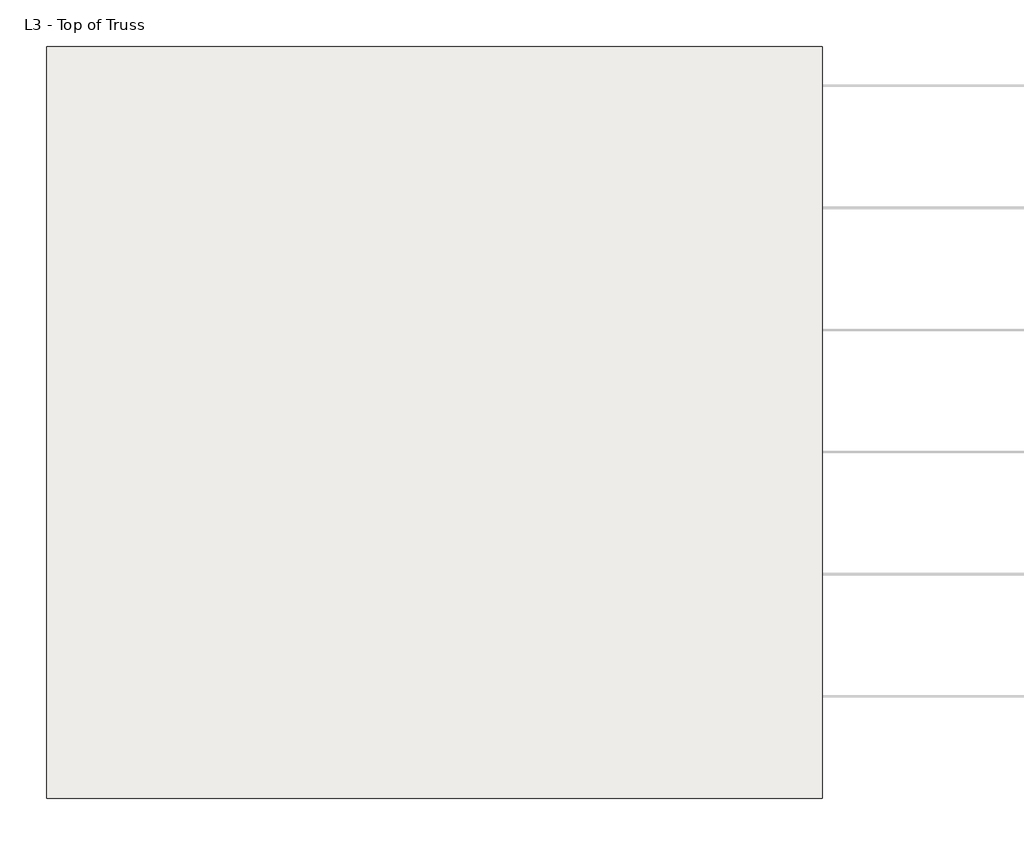
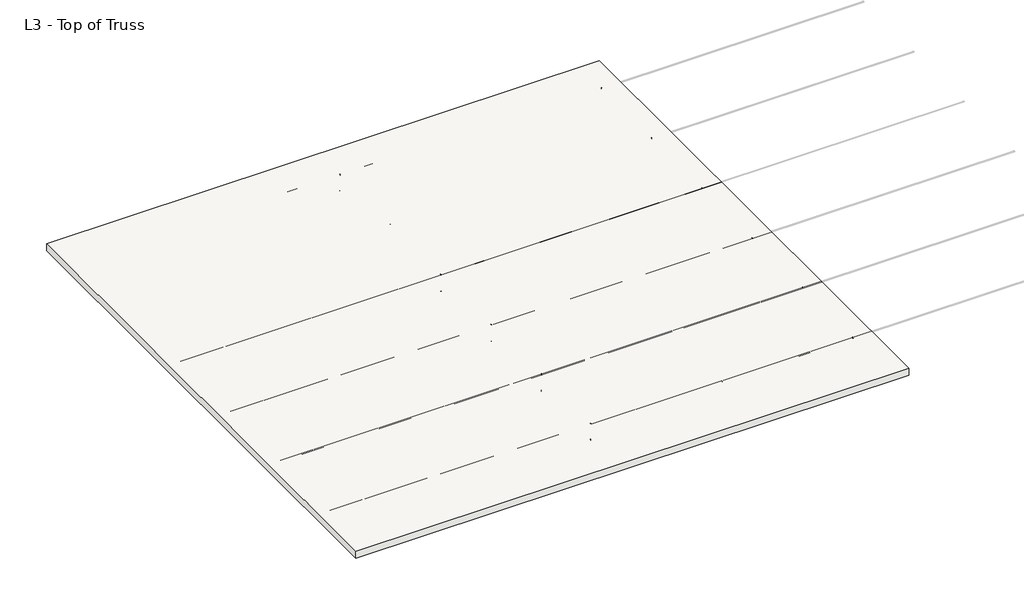
# One storey, part 1 of 2: 98 beams, 1 roof.
"""IFC4 building model written with IfcOpenShell, lengths in millimetres."""

import ifcopenshell
import ifcopenshell.guid

model = None  # the IFC model being written
_history = None  # IfcOwnerHistory: only IFC2X3 demands one
_inside = {}  # id of a spatial element -> (the spatial element, [elements in it])
_under = {}  # id of a project, library or spatial element -> (it, [spatial elements below it])
_declared = {}  # id of a project -> (the project, [libraries it declares])
_typed = {}  # id of a type object -> (the type object, [elements of that type])
_made_of = {}  # id of a material, layer set ... -> (it, [elements and type objects made of it])


def new_model(schema):
    """Start an empty IFC model of exactly this schema.

    Asked for "IFC4X3", IfcOpenShell would pick the latest addendum, in which some entities
    have other attributes; the version numbers below select the first issue.
    IFC2X3 requires an IfcOwnerHistory on every rooted entity: one is made here for all.
    """
    global model, _history
    if schema == "IFC4X3":
        model = ifcopenshell.file(schema_version=(4, 3, 0, 0))
    else:
        model = ifcopenshell.file(schema=schema)
    _inside.clear()
    _under.clear()
    _declared.clear()
    _typed.clear()
    _made_of.clear()
    _history = None
    if model.schema == "IFC2X3":
        org = make("IfcOrganization", Name="unknown")
        user = make(
            "IfcPersonAndOrganization",
            ThePerson=make("IfcPerson", FamilyName="unknown"),
            TheOrganization=org,
        )
        app = make(
            "IfcApplication",
            ApplicationDeveloper=org,
            Version="unknown",
            ApplicationFullName="unknown",
            ApplicationIdentifier="unknown",
        )
        _history = make(
            "IfcOwnerHistory",
            OwningUser=user,
            OwningApplication=app,
            ChangeAction="ADDED",
            CreationDate=0,
        )
    return model


def make(cls, **values):
    """One entity of the class cls with the attributes given. An attribute that is None is left unset."""
    return model.create_entity(
        cls, **{name: value for name, value in values.items() if value is not None}
    )


def rooted(cls, **values):
    """An entity with a GlobalId (a new one), such as an element, a storey or a relation."""
    return make(cls, GlobalId=ifcopenshell.guid.new(), OwnerHistory=_history, **values)


def si_unit(unit_type, name, prefix=None):
    """IfcSIUnit, for example si_unit("LENGTHUNIT", "METRE", prefix="MILLI")."""
    return make("IfcSIUnit", UnitType=unit_type, Prefix=prefix, Name=name)


def assignment(units):
    """IfcUnitAssignment: the units of a project."""
    return None if units is None else make("IfcUnitAssignment", Units=units)


def point(xyz):
    """IfcCartesianPoint."""
    return None if xyz is None else make("IfcCartesianPoint", Coordinates=xyz)


def direction(xyz):
    """IfcDirection."""
    return None if xyz is None else make("IfcDirection", DirectionRatios=xyz)


def frame(location, z_axis=None, x_axis=None):
    """IfcAxis2Placement3D, a coordinate frame: its origin and axes. An axis left out is left unset."""
    return make(
        "IfcAxis2Placement3D",
        Location=point(location),
        Axis=direction(z_axis),
        RefDirection=direction(x_axis),
    )


def frame_2d(location, x_axis=None):
    """IfcAxis2Placement2D, a coordinate frame in the plane: its origin and x axis."""
    return make(
        "IfcAxis2Placement2D", Location=point(location), RefDirection=direction(x_axis)
    )


def origin():
    """The frame at (0, 0, 0) with its axes left unset."""
    return frame((0.0, 0.0, 0.0))


def origin_2d():
    """The frame at (0, 0) in the plane with its x axis left unset."""
    return frame_2d((0.0, 0.0))


def place(relative_to, where):
    """IfcLocalPlacement: puts the frame where relative to a parent placement (None: the world)."""
    return make(
        "IfcLocalPlacement", PlacementRelTo=relative_to, RelativePlacement=where
    )


def context(
    kind, dimensions, precision=None, world=None, true_north=None, identifier=None
):
    """IfcGeometricRepresentationContext, for example the 3D "Model" context."""
    return make(
        "IfcGeometricRepresentationContext",
        ContextIdentifier=identifier,
        ContextType=kind,
        CoordinateSpaceDimension=dimensions,
        Precision=precision,
        WorldCoordinateSystem=world,
        TrueNorth=true_north,
    )


def project(units=None, contexts=None):
    """IfcProject with its units and contexts."""
    return rooted(
        "IfcProject",
        Name="project",
        RepresentationContexts=contexts,
        UnitsInContext=assignment(units),
    )


def spatial(cls, under=None, at=None, **own):
    """A site, building, storey or space (cls), placed at a placement, below another one or the project."""
    s = rooted(cls, ObjectPlacement=at, **own)
    if under is not None:
        _under.setdefault(under.id(), (under, []))[1].append(s)
    return s


def polyline(points):
    """IfcPolyline through the points."""
    return make("IfcPolyline", Points=[point(p) for p in points])


def circle_curve(where, radius):
    """IfcCircle in the frame where."""
    return make("IfcCircle", Position=where, Radius=radius)


def trimmed(basis, trim1, trim2, sense, master):
    """IfcTrimmedCurve: the piece of a basis curve between two trims."""
    return make(
        "IfcTrimmedCurve",
        BasisCurve=basis,
        Trim1=trim1,
        Trim2=trim2,
        SenseAgreement=sense,
        MasterRepresentation=master,
    )


def segment(curve, same_sense, transition):
    """IfcCompositeCurveSegment."""
    return make(
        "IfcCompositeCurveSegment",
        Transition=transition,
        SameSense=same_sense,
        ParentCurve=curve,
    )


def composite_curve(segments, self_intersect=None):
    """IfcCompositeCurve: segments joined end to end."""
    return make("IfcCompositeCurve", Segments=segments, SelfIntersect=self_intersect)


def outline(outer, holes=None, kind="AREA"):
    """IfcArbitraryClosedProfileDef: a profile drawn as a closed curve; with holes, ...WithVoids."""
    if holes is None:
        return make("IfcArbitraryClosedProfileDef", ProfileType=kind, OuterCurve=outer)
    return make(
        "IfcArbitraryProfileDefWithVoids",
        ProfileType=kind,
        OuterCurve=outer,
        InnerCurves=holes,
    )


def extrude(swept, where, along, depth):
    """IfcExtrudedAreaSolid: the profile swept, set in the frame where, extruded along a direction by depth."""
    return make(
        "IfcExtrudedAreaSolid",
        SweptArea=swept,
        Position=where,
        ExtrudedDirection=direction(along),
        Depth=depth,
    )


def shape(context_of_items, identifier, shape_type, items):
    """IfcShapeRepresentation: the items that make up one representation, for example the "Body"."""
    return make(
        "IfcShapeRepresentation",
        ContextOfItems=context_of_items,
        RepresentationIdentifier=identifier,
        RepresentationType=shape_type,
        Items=items,
    )


def source(mapping_origin, context_of_items, identifier, shape_type, items):
    """IfcRepresentationMap: a shape defined once, which mapped items show again and again."""
    return make(
        "IfcRepresentationMap",
        MappingOrigin=mapping_origin,
        MappedRepresentation=shape(context_of_items, identifier, shape_type, items),
    )


def transform(
    local_origin,
    x_axis=None,
    y_axis=None,
    z_axis=None,
    scale=None,
    scale2=None,
    scale3=None,
    uniform=True,
):
    """IfcCartesianTransformationOperator3D, or its non-uniform kind. x_axis, y_axis, z_axis: its Axis1, 2, 3."""
    if uniform:
        return make(
            "IfcCartesianTransformationOperator3D",
            Axis1=direction(x_axis),
            Axis2=direction(y_axis),
            LocalOrigin=point(local_origin),
            Scale=scale,
            Axis3=direction(z_axis),
        )
    return make(
        "IfcCartesianTransformationOperator3DnonUniform",
        Axis1=direction(x_axis),
        Axis2=direction(y_axis),
        LocalOrigin=point(local_origin),
        Scale=scale,
        Axis3=direction(z_axis),
        Scale2=scale2,
        Scale3=scale3,
    )


def mapped(mapping_source, mapping_target):
    """IfcMappedItem: shows the shape of a source again, moved by a transform."""
    return make(
        "IfcMappedItem", MappingSource=mapping_source, MappingTarget=mapping_target
    )


def made_of(thing, what):
    """Note that an element or type object is made of a material, layer set ...; save() writes the relation."""
    if what is not None:
        _made_of.setdefault(what.id(), (what, []))[1].append(thing)
    return thing


def element(
    cls,
    number,
    at=None,
    inside=None,
    cuts=None,
    type_object=None,
    material=None,
    context=None,
    identifier="Body",
    shape_type=None,
    held_by="IfcProductDefinitionShape",
    body=None,
    shapes=None,
    **own,
):
    """One element of the class cls, such as IfcWall. Its Tag is "e" and its number.

    at: its placement. inside: the storey or other place that contains it. cuts: it is an
    opening in that element (IfcRelVoidsElement). A single representation is given by context,
    identifier, shape_type and body (its items); several are given by shapes. held_by: the class
    of the entity that holds the representations. save() writes the other relations.
    """
    e = rooted(cls, Tag="e%d" % number, ObjectPlacement=at, **own)
    if body is not None:
        shapes = [shape(context, identifier, shape_type, body)]
    if shapes is not None:
        e.Representation = make(held_by, Representations=shapes)
    if inside is not None:
        _inside.setdefault(inside.id(), (inside, []))[1].append(e)
    if cuts is not None:
        rooted(
            "IfcRelVoidsElement", RelatingBuildingElement=cuts, RelatedOpeningElement=e
        )
    if type_object is not None:
        _typed.setdefault(type_object.id(), (type_object, []))[1].append(e)
    return made_of(e, material)


def aggregate(whole, parts):
    """IfcRelAggregates: a whole, such as a stair, and the parts it consists of."""
    return rooted("IfcRelAggregates", RelatingObject=whole, RelatedObjects=parts)


def save(model, path):
    """Write the relations noted so far, then the file.

    IfcRelAggregates (storeys below a building ...), IfcRelContainedInSpatialStructure (elements
    in a storey), IfcRelDefinesByType, IfcRelAssociatesMaterial and IfcRelDeclares: one each for
    every whole, place, type object, material and project.
    """
    for whole, parts in _under.values():
        aggregate(whole, parts)
    for where, things in _inside.values():
        rooted(
            "IfcRelContainedInSpatialStructure",
            RelatedElements=things,
            RelatingStructure=where,
        )
    for kind, things in _typed.values():
        rooted("IfcRelDefinesByType", RelatedObjects=things, RelatingType=kind)
    for what, things in _made_of.values():
        rooted("IfcRelAssociatesMaterial", RelatedObjects=things, RelatingMaterial=what)
    for by, libraries in _declared.values():
        rooted("IfcRelDeclares", RelatingContext=by, RelatedDefinitions=libraries)
    model.write(path)


def circular_hollow_sections_chs60_3x5_c94bd862(model_context):
    return source(origin(), model_context, "Body", "SweptSolid", [
        extrude(outline(composite_curve([segment(trimmed(circle_curve(origin_2d(), 30.15), [point((-30.15, 0.0))], [point((30.15, 0.0))], False, "CARTESIAN"), True, "CONTINUOUS"), segment(trimmed(circle_curve(origin_2d(), 30.15), [point((30.15, 0.0))], [point((-30.15, 0.0))], False, "CARTESIAN"), True, "CONTINUOUS")], self_intersect=False), holes=[composite_curve([segment(trimmed(circle_curve(origin_2d(), 25.15), [point((25.15, 0.0))], [point((-25.15, 0.0))], True, "CARTESIAN"), True, "CONTINUOUS"), segment(trimmed(circle_curve(origin_2d(), 25.15), [point((-25.15, 0.0))], [point((25.15, 0.0))], True, "CARTESIAN"), True, "CONTINUOUS")], self_intersect=False)]), frame((-557.0, 0.0, 0.0), z_axis=(1.0, 0.0, 0.0), x_axis=(0.0, 1.0, 0.0)), (0.0, 0.0, 1.0), 1114.0),
    ])


def circular_hollow_sections_chs60_3x5_b8a643cb(model_context):
    return source(origin(), model_context, "Body", "SweptSolid", [
        extrude(outline(composite_curve([segment(trimmed(circle_curve(origin_2d(), 30.15), [point((-30.15, 0.0))], [point((30.15, 0.0))], False, "CARTESIAN"), True, "CONTINUOUS"), segment(trimmed(circle_curve(origin_2d(), 30.15), [point((30.15, 0.0))], [point((-30.15, 0.0))], False, "CARTESIAN"), True, "CONTINUOUS")], self_intersect=False), holes=[composite_curve([segment(trimmed(circle_curve(origin_2d(), 25.15), [point((25.15, 0.0))], [point((-25.15, 0.0))], True, "CARTESIAN"), True, "CONTINUOUS"), segment(trimmed(circle_curve(origin_2d(), 25.15), [point((-25.15, 0.0))], [point((25.15, 0.0))], True, "CARTESIAN"), True, "CONTINUOUS")], self_intersect=False)]), frame((-790.0, 0.0, 0.0), z_axis=(1.0, 0.0, 0.0), x_axis=(0.0, 1.0, 0.0)), (0.0, 0.0, 1.0), 1580.0),
    ])


def circular_hollow_sections_chs60_3x5_ee2473de(model_context):
    return source(origin(), model_context, "Body", "SweptSolid", [
        extrude(outline(composite_curve([segment(trimmed(circle_curve(origin_2d(), 30.15), [point((-30.15, 0.0))], [point((30.15, 0.0))], False, "CARTESIAN"), True, "CONTINUOUS"), segment(trimmed(circle_curve(origin_2d(), 30.15), [point((30.15, 0.0))], [point((-30.15, 0.0))], False, "CARTESIAN"), True, "CONTINUOUS")], self_intersect=False), holes=[composite_curve([segment(trimmed(circle_curve(origin_2d(), 25.15), [point((25.15, 0.0))], [point((-25.15, 0.0))], True, "CARTESIAN"), True, "CONTINUOUS"), segment(trimmed(circle_curve(origin_2d(), 25.15), [point((-25.15, 0.0))], [point((25.15, 0.0))], True, "CARTESIAN"), True, "CONTINUOUS")], self_intersect=False)]), frame((-9000.0, 0.0, 0.0), z_axis=(1.0, 0.0, 0.0), x_axis=(0.0, 1.0, 0.0)), (0.0, 0.0, 1.0), 18000.0),
    ])


def circular_hollow_sections_chs60_3x5_7809bf4e(model_context):
    return source(origin(), model_context, "Body", "SweptSolid", [
        extrude(outline(composite_curve([segment(trimmed(circle_curve(origin_2d(), 30.15), [point((-30.15, 0.0))], [point((30.15, 0.0))], False, "CARTESIAN"), True, "CONTINUOUS"), segment(trimmed(circle_curve(origin_2d(), 30.15), [point((30.15, 0.0))], [point((-30.15, 0.0))], False, "CARTESIAN"), True, "CONTINUOUS")], self_intersect=False), holes=[composite_curve([segment(trimmed(circle_curve(origin_2d(), 25.15), [point((25.15, 0.0))], [point((-25.15, 0.0))], True, "CARTESIAN"), True, "CONTINUOUS"), segment(trimmed(circle_curve(origin_2d(), 25.15), [point((-25.15, 0.0))], [point((25.15, 0.0))], True, "CARTESIAN"), True, "CONTINUOUS")], self_intersect=False)]), frame((-600.0, 0.0, 0.0), z_axis=(1.0, 0.0, 0.0), x_axis=(0.0, 1.0, 0.0)), (0.0, 0.0, 1.0), 1157.0),
    ])


model = new_model("IFC4")

# Units and contexts
model_context = context("Model", 3, world=origin())
ifc_project = project(units=[si_unit("LENGTHUNIT", "METRE", prefix="MILLI")], contexts=[model_context])

# Site, building, storey
site = spatial("IfcSite", under=ifc_project)
building = spatial("IfcBuilding", under=site)
storey = spatial("IfcBuildingStorey", under=building, Name="L3 - Top of Truss", Elevation=7800.0)

# Beams
placement = place(None, origin())
circular_hollow_sections_chs60_3x5_shape = circular_hollow_sections_chs60_3x5_c94bd862(model_context)
element("IfcBeam", 1, ObjectType="Circular Hollow Sections : CHS60.3x5", at=placement, inside=storey, context=model_context, shape_type="MappedRepresentation", body=[
    mapped(circular_hollow_sections_chs60_3x5_shape, transform((-5853.84106, -5058.7619082, 7200.0), x_axis=(0.0, 0.0, 1.0), y_axis=(0.0, -1.0, 0.0), z_axis=(1.0, 0.0, 0.0))),
])
element("IfcBeam", 2, ObjectType="Circular Hollow Sections : CHS60.3x5", at=placement, inside=storey, context=model_context, shape_type="MappedRepresentation", body=[
    mapped(circular_hollow_sections_chs60_3x5_shape, transform((-4568.1267743, -5058.7619082, 7200.0), x_axis=(0.0, 0.0, 1.0), y_axis=(0.0, -1.0, 0.0), z_axis=(1.0, 0.0, 0.0))),
])
element("IfcBeam", 3, ObjectType="Circular Hollow Sections : CHS60.3x5", at=placement, inside=storey, context=model_context, shape_type="MappedRepresentation", body=[
    mapped(circular_hollow_sections_chs60_3x5_shape, transform((-3282.4124885, -5058.7619082, 7200.0), x_axis=(0.0, 0.0, 1.0), y_axis=(0.0, -1.0, 0.0), z_axis=(1.0, 0.0, 0.0))),
])
element("IfcBeam", 4, ObjectType="Circular Hollow Sections : CHS60.3x5", at=placement, inside=storey, context=model_context, shape_type="MappedRepresentation", body=[
    mapped(circular_hollow_sections_chs60_3x5_shape, transform((-1996.6982028, -5058.7619082, 7200.0), x_axis=(0.0, 0.0, 1.0), y_axis=(0.0, -1.0, 0.0), z_axis=(1.0, 0.0, 0.0))),
])
element("IfcBeam", 5, ObjectType="Circular Hollow Sections : CHS60.3x5", at=placement, inside=storey, context=model_context, shape_type="MappedRepresentation", body=[
    mapped(circular_hollow_sections_chs60_3x5_shape, transform((-710.9839171, -5058.7619082, 7200.0), x_axis=(0.0, 0.0, 1.0), y_axis=(0.0, -1.0, 0.0), z_axis=(1.0, 0.0, 0.0))),
])
element("IfcBeam", 6, ObjectType="Circular Hollow Sections : CHS60.3x5", at=placement, inside=storey, context=model_context, shape_type="MappedRepresentation", body=[
    mapped(circular_hollow_sections_chs60_3x5_shape, transform((-5853.84106, -11058.7619082, 7200.0), x_axis=(0.0, 0.0, 1.0), y_axis=(0.0, -1.0, 0.0), z_axis=(1.0, 0.0, 0.0))),
])
element("IfcBeam", 7, ObjectType="Circular Hollow Sections : CHS60.3x5", at=placement, inside=storey, context=model_context, shape_type="MappedRepresentation", body=[
    mapped(circular_hollow_sections_chs60_3x5_shape, transform((-4568.1267743, -11058.7619082, 7200.0), x_axis=(0.0, 0.0, 1.0), y_axis=(0.0, -1.0, 0.0), z_axis=(1.0, 0.0, 0.0))),
])
element("IfcBeam", 8, ObjectType="Circular Hollow Sections : CHS60.3x5", at=placement, inside=storey, context=model_context, shape_type="MappedRepresentation", body=[
    mapped(circular_hollow_sections_chs60_3x5_shape, transform((-3282.4124885, -11058.7619082, 7200.0), x_axis=(0.0, 0.0, 1.0), y_axis=(0.0, -1.0, 0.0), z_axis=(1.0, 0.0, 0.0))),
])
element("IfcBeam", 9, ObjectType="Circular Hollow Sections : CHS60.3x5", at=placement, inside=storey, context=model_context, shape_type="MappedRepresentation", body=[
    mapped(circular_hollow_sections_chs60_3x5_shape, transform((5717.5875115, -11058.7619082, 7200.0), x_axis=(0.0, 0.0, 1.0), y_axis=(0.0, -1.0, 0.0), z_axis=(1.0, 0.0, 0.0))),
])
element("IfcBeam", 10, ObjectType="Circular Hollow Sections : CHS60.3x5", at=placement, inside=storey, context=model_context, shape_type="MappedRepresentation", body=[
    mapped(circular_hollow_sections_chs60_3x5_shape, transform((4431.8732257, -11058.7619082, 7200.0), x_axis=(0.0, 0.0, 1.0), y_axis=(0.0, -1.0, 0.0), z_axis=(1.0, 0.0, 0.0))),
])
element("IfcBeam", 11, ObjectType="Circular Hollow Sections : CHS60.3x5", at=placement, inside=storey, context=model_context, shape_type="MappedRepresentation", body=[
    mapped(circular_hollow_sections_chs60_3x5_shape, transform((3146.15894, -11058.7619082, 7200.0), x_axis=(0.0, 0.0, 1.0), y_axis=(0.0, -1.0, 0.0), z_axis=(1.0, 0.0, 0.0))),
])
element("IfcBeam", 12, ObjectType="Circular Hollow Sections : CHS60.3x5", at=placement, inside=storey, context=model_context, shape_type="MappedRepresentation", body=[
    mapped(circular_hollow_sections_chs60_3x5_shape, transform((-1996.6982028, -11058.7619082, 7200.0), x_axis=(0.0, 0.0, 1.0), y_axis=(0.0, -1.0, 0.0), z_axis=(1.0, 0.0, 0.0))),
])
element("IfcBeam", 13, ObjectType="Circular Hollow Sections : CHS60.3x5", at=placement, inside=storey, context=model_context, shape_type="MappedRepresentation", body=[
    mapped(circular_hollow_sections_chs60_3x5_shape, transform((-710.9839171, -11058.7619082, 7200.0), x_axis=(0.0, 0.0, 1.0), y_axis=(0.0, -1.0, 0.0), z_axis=(1.0, 0.0, 0.0))),
])
element("IfcBeam", 14, ObjectType="Circular Hollow Sections : CHS60.3x5", at=placement, inside=storey, context=model_context, shape_type="MappedRepresentation", body=[
    mapped(circular_hollow_sections_chs60_3x5_shape, transform((574.7303686, -11058.7619082, 7200.0), x_axis=(0.0, 0.0, 1.0), y_axis=(0.0, -1.0, 0.0), z_axis=(1.0, 0.0, 0.0))),
])
element("IfcBeam", 15, ObjectType="Circular Hollow Sections : CHS60.3x5", at=placement, inside=storey, context=model_context, shape_type="MappedRepresentation", body=[
    mapped(circular_hollow_sections_chs60_3x5_shape, transform((1860.4446543, -11058.7619082, 7200.0), x_axis=(0.0, 0.0, 1.0), y_axis=(0.0, -1.0, 0.0), z_axis=(1.0, 0.0, 0.0))),
])
element("IfcBeam", 16, ObjectType="Circular Hollow Sections : CHS60.3x5", at=placement, inside=storey, context=model_context, shape_type="MappedRepresentation", body=[
    mapped(circular_hollow_sections_chs60_3x5_shape, transform((9574.7303686, -17058.7619082, 7200.0), x_axis=(0.0, 0.0, 1.0), y_axis=(0.0, -1.0, 0.0), z_axis=(1.0, 0.0, 0.0))),
])
element("IfcBeam", 17, ObjectType="Circular Hollow Sections : CHS60.3x5", at=placement, inside=storey, context=model_context, shape_type="MappedRepresentation", body=[
    mapped(circular_hollow_sections_chs60_3x5_shape, transform((-5853.84106, -17058.7619082, 7200.0), x_axis=(0.0, 0.0, 1.0), y_axis=(0.0, -1.0, 0.0), z_axis=(1.0, 0.0, 0.0))),
])
element("IfcBeam", 18, ObjectType="Circular Hollow Sections : CHS60.3x5", at=placement, inside=storey, context=model_context, shape_type="MappedRepresentation", body=[
    mapped(circular_hollow_sections_chs60_3x5_shape, transform((8289.0160829, -17058.7619082, 7200.0), x_axis=(0.0, 0.0, 1.0), y_axis=(0.0, -1.0, 0.0), z_axis=(1.0, 0.0, 0.0))),
])
element("IfcBeam", 19, ObjectType="Circular Hollow Sections : CHS60.3x5", at=placement, inside=storey, context=model_context, shape_type="MappedRepresentation", body=[
    mapped(circular_hollow_sections_chs60_3x5_shape, transform((-4568.1267743, -17058.7619082, 7200.0), x_axis=(0.0, 0.0, 1.0), y_axis=(0.0, -1.0, 0.0), z_axis=(1.0, 0.0, 0.0))),
])
element("IfcBeam", 20, ObjectType="Circular Hollow Sections : CHS60.3x5", at=placement, inside=storey, context=model_context, shape_type="MappedRepresentation", body=[
    mapped(circular_hollow_sections_chs60_3x5_shape, transform((7003.3017972, -17058.7619082, 7200.0), x_axis=(0.0, 0.0, 1.0), y_axis=(0.0, -1.0, 0.0), z_axis=(1.0, 0.0, 0.0))),
])
element("IfcBeam", 21, ObjectType="Circular Hollow Sections : CHS60.3x5", at=placement, inside=storey, context=model_context, shape_type="MappedRepresentation", body=[
    mapped(circular_hollow_sections_chs60_3x5_shape, transform((-3282.4124885, -17058.7619082, 7200.0), x_axis=(0.0, 0.0, 1.0), y_axis=(0.0, -1.0, 0.0), z_axis=(1.0, 0.0, 0.0))),
])
element("IfcBeam", 22, ObjectType="Circular Hollow Sections : CHS60.3x5", at=placement, inside=storey, context=model_context, shape_type="MappedRepresentation", body=[
    mapped(circular_hollow_sections_chs60_3x5_shape, transform((5717.5875115, -17058.7619082, 7200.0), x_axis=(0.0, 0.0, 1.0), y_axis=(0.0, -1.0, 0.0), z_axis=(1.0, 0.0, 0.0))),
])
element("IfcBeam", 23, ObjectType="Circular Hollow Sections : CHS60.3x5", at=placement, inside=storey, context=model_context, shape_type="MappedRepresentation", body=[
    mapped(circular_hollow_sections_chs60_3x5_shape, transform((4431.8732257, -17058.7619082, 7200.0), x_axis=(0.0, 0.0, 1.0), y_axis=(0.0, -1.0, 0.0), z_axis=(1.0, 0.0, 0.0))),
])
element("IfcBeam", 24, ObjectType="Circular Hollow Sections : CHS60.3x5", at=placement, inside=storey, context=model_context, shape_type="MappedRepresentation", body=[
    mapped(circular_hollow_sections_chs60_3x5_shape, transform((3146.15894, -17058.7619082, 7200.0), x_axis=(0.0, 0.0, 1.0), y_axis=(0.0, -1.0, 0.0), z_axis=(1.0, 0.0, 0.0))),
])
element("IfcBeam", 25, ObjectType="Circular Hollow Sections : CHS60.3x5", at=placement, inside=storey, context=model_context, shape_type="MappedRepresentation", body=[
    mapped(circular_hollow_sections_chs60_3x5_shape, transform((-1996.6982028, -17058.7619082, 7200.0), x_axis=(0.0, 0.0, 1.0), y_axis=(0.0, -1.0, 0.0), z_axis=(1.0, 0.0, 0.0))),
])
element("IfcBeam", 26, ObjectType="Circular Hollow Sections : CHS60.3x5", at=placement, inside=storey, context=model_context, shape_type="MappedRepresentation", body=[
    mapped(circular_hollow_sections_chs60_3x5_shape, transform((-710.9839171, -17058.7619082, 7200.0), x_axis=(0.0, 0.0, 1.0), y_axis=(0.0, -1.0, 0.0), z_axis=(1.0, 0.0, 0.0))),
])
element("IfcBeam", 27, ObjectType="Circular Hollow Sections : CHS60.3x5", at=placement, inside=storey, context=model_context, shape_type="MappedRepresentation", body=[
    mapped(circular_hollow_sections_chs60_3x5_shape, transform((574.7303686, -17058.7619082, 7200.0), x_axis=(0.0, 0.0, 1.0), y_axis=(0.0, -1.0, 0.0), z_axis=(1.0, 0.0, 0.0))),
])
element("IfcBeam", 28, ObjectType="Circular Hollow Sections : CHS60.3x5", at=placement, inside=storey, context=model_context, shape_type="MappedRepresentation", body=[
    mapped(circular_hollow_sections_chs60_3x5_shape, transform((1860.4446543, -17058.7619082, 7200.0), x_axis=(0.0, 0.0, 1.0), y_axis=(0.0, -1.0, 0.0), z_axis=(1.0, 0.0, 0.0))),
])
element("IfcBeam", 29, ObjectType="Circular Hollow Sections : CHS60.3x5", at=placement, inside=storey, context=model_context, shape_type="MappedRepresentation", body=[
    mapped(circular_hollow_sections_chs60_3x5_shape, transform((9574.7303686, -22948.7619082, 7200.0), x_axis=(0.0, 0.0, 1.0), y_axis=(0.0, -1.0, 0.0), z_axis=(1.0, 0.0, 0.0))),
])
element("IfcBeam", 30, ObjectType="Circular Hollow Sections : CHS60.3x5", at=placement, inside=storey, context=model_context, shape_type="MappedRepresentation", body=[
    mapped(circular_hollow_sections_chs60_3x5_shape, transform((-5853.84106, -22948.7619082, 7200.0), x_axis=(0.0, 0.0, 1.0), y_axis=(0.0, -1.0, 0.0), z_axis=(1.0, 0.0, 0.0))),
])
element("IfcBeam", 31, ObjectType="Circular Hollow Sections : CHS60.3x5", at=placement, inside=storey, context=model_context, shape_type="MappedRepresentation", body=[
    mapped(circular_hollow_sections_chs60_3x5_shape, transform((8289.0160829, -22948.7619082, 7200.0), x_axis=(0.0, 0.0, 1.0), y_axis=(0.0, -1.0, 0.0), z_axis=(1.0, 0.0, 0.0))),
])
element("IfcBeam", 32, ObjectType="Circular Hollow Sections : CHS60.3x5", at=placement, inside=storey, context=model_context, shape_type="MappedRepresentation", body=[
    mapped(circular_hollow_sections_chs60_3x5_shape, transform((-4568.1267743, -22948.7619082, 7200.0), x_axis=(0.0, 0.0, 1.0), y_axis=(0.0, -1.0, 0.0), z_axis=(1.0, 0.0, 0.0))),
])
element("IfcBeam", 33, ObjectType="Circular Hollow Sections : CHS60.3x5", at=placement, inside=storey, context=model_context, shape_type="MappedRepresentation", body=[
    mapped(circular_hollow_sections_chs60_3x5_shape, transform((7003.3017972, -22948.7619082, 7200.0), x_axis=(0.0, 0.0, 1.0), y_axis=(0.0, -1.0, 0.0), z_axis=(1.0, 0.0, 0.0))),
])
element("IfcBeam", 34, ObjectType="Circular Hollow Sections : CHS60.3x5", at=placement, inside=storey, context=model_context, shape_type="MappedRepresentation", body=[
    mapped(circular_hollow_sections_chs60_3x5_shape, transform((-3282.4124885, -22948.7619082, 7200.0), x_axis=(0.0, 0.0, 1.0), y_axis=(0.0, -1.0, 0.0), z_axis=(1.0, 0.0, 0.0))),
])
element("IfcBeam", 35, ObjectType="Circular Hollow Sections : CHS60.3x5", at=placement, inside=storey, context=model_context, shape_type="MappedRepresentation", body=[
    mapped(circular_hollow_sections_chs60_3x5_shape, transform((5717.5875115, -22948.7619082, 7200.0), x_axis=(0.0, 0.0, 1.0), y_axis=(0.0, -1.0, 0.0), z_axis=(1.0, 0.0, 0.0))),
])
element("IfcBeam", 36, ObjectType="Circular Hollow Sections : CHS60.3x5", at=placement, inside=storey, context=model_context, shape_type="MappedRepresentation", body=[
    mapped(circular_hollow_sections_chs60_3x5_shape, transform((4431.8732257, -22948.7619082, 7200.0), x_axis=(0.0, 0.0, 1.0), y_axis=(0.0, -1.0, 0.0), z_axis=(1.0, 0.0, 0.0))),
])
element("IfcBeam", 37, ObjectType="Circular Hollow Sections : CHS60.3x5", at=placement, inside=storey, context=model_context, shape_type="MappedRepresentation", body=[
    mapped(circular_hollow_sections_chs60_3x5_shape, transform((10860.4446543, -22948.7619082, 7200.0), x_axis=(0.0, 0.0, 1.0), y_axis=(0.0, -1.0, 0.0), z_axis=(1.0, 0.0, 0.0))),
])
element("IfcBeam", 38, ObjectType="Circular Hollow Sections : CHS60.3x5", at=placement, inside=storey, context=model_context, shape_type="MappedRepresentation", body=[
    mapped(circular_hollow_sections_chs60_3x5_shape, transform((3146.15894, -22948.7619082, 7200.0), x_axis=(0.0, 0.0, 1.0), y_axis=(0.0, -1.0, 0.0), z_axis=(1.0, 0.0, 0.0))),
])
element("IfcBeam", 39, ObjectType="Circular Hollow Sections : CHS60.3x5", at=placement, inside=storey, context=model_context, shape_type="MappedRepresentation", body=[
    mapped(circular_hollow_sections_chs60_3x5_shape, transform((-1996.6982028, -22948.7619082, 7200.0), x_axis=(0.0, 0.0, 1.0), y_axis=(0.0, -1.0, 0.0), z_axis=(1.0, 0.0, 0.0))),
])
element("IfcBeam", 40, ObjectType="Circular Hollow Sections : CHS60.3x5", at=placement, inside=storey, context=model_context, shape_type="MappedRepresentation", body=[
    mapped(circular_hollow_sections_chs60_3x5_shape, transform((-710.9839171, -22948.7619082, 7200.0), x_axis=(0.0, 0.0, 1.0), y_axis=(0.0, -1.0, 0.0), z_axis=(1.0, 0.0, 0.0))),
])
element("IfcBeam", 41, ObjectType="Circular Hollow Sections : CHS60.3x5", at=placement, inside=storey, context=model_context, shape_type="MappedRepresentation", body=[
    mapped(circular_hollow_sections_chs60_3x5_shape, transform((-7139.5553457, -22948.7619082, 7200.0), x_axis=(0.0, 0.0, 1.0), y_axis=(0.0, -1.0, 0.0), z_axis=(1.0, 0.0, 0.0))),
])
element("IfcBeam", 42, ObjectType="Circular Hollow Sections : CHS60.3x5", at=placement, inside=storey, context=model_context, shape_type="MappedRepresentation", body=[
    mapped(circular_hollow_sections_chs60_3x5_shape, transform((574.7303686, -22948.7619082, 7200.0), x_axis=(0.0, 0.0, 1.0), y_axis=(0.0, -1.0, 0.0), z_axis=(1.0, 0.0, 0.0))),
])
element("IfcBeam", 43, ObjectType="Circular Hollow Sections : CHS60.3x5", at=placement, inside=storey, context=model_context, shape_type="MappedRepresentation", body=[
    mapped(circular_hollow_sections_chs60_3x5_shape, transform((1860.4446543, -22948.7619082, 7200.0), x_axis=(0.0, 0.0, 1.0), y_axis=(0.0, -1.0, 0.0), z_axis=(1.0, 0.0, 0.0))),
])
circular_hollow_sections_chs60_3x5_2_shape = circular_hollow_sections_chs60_3x5_b8a643cb(model_context)
element("IfcBeam", 44, ObjectType="Circular Hollow Sections : CHS60.3x5", at=placement, inside=storey, context=model_context, shape_type="MappedRepresentation", body=[
    mapped(circular_hollow_sections_chs60_3x5_2_shape, transform((-5210.9839171, -5058.7619082, 7200.0), x_axis=(0.7310552682428689, 0.0, -0.6823182503600113), y_axis=(0.0, -1.0, 0.0), z_axis=(-0.6823182503600113, 0.0, -0.7310552682428689))),
])
element("IfcBeam", 45, ObjectType="Circular Hollow Sections : CHS60.3x5", at=placement, inside=storey, context=model_context, shape_type="MappedRepresentation", body=[
    mapped(circular_hollow_sections_chs60_3x5_2_shape, transform((-3925.2696314, -5058.7619082, 7200.0), x_axis=(0.7310552682428689, 0.0, -0.6823182503600113), y_axis=(0.0, -1.0, 0.0), z_axis=(-0.6823182503600113, 0.0, -0.7310552682428689))),
])
element("IfcBeam", 46, ObjectType="Circular Hollow Sections : CHS60.3x5", at=placement, inside=storey, context=model_context, shape_type="MappedRepresentation", body=[
    mapped(circular_hollow_sections_chs60_3x5_2_shape, transform((-2639.5553457, -5058.7619082, 7200.0), x_axis=(0.7310552682428689, 0.0, -0.6823182503600113), y_axis=(0.0, -1.0, 0.0), z_axis=(-0.6823182503600113, 0.0, -0.7310552682428689))),
])
element("IfcBeam", 47, ObjectType="Circular Hollow Sections : CHS60.3x5", at=placement, inside=storey, context=model_context, shape_type="MappedRepresentation", body=[
    mapped(circular_hollow_sections_chs60_3x5_2_shape, transform((-1353.84106, -5058.7619082, 7200.0), x_axis=(0.7310552682428689, 0.0, -0.6823182503600113), y_axis=(0.0, -1.0, 0.0), z_axis=(-0.6823182503600113, 0.0, -0.7310552682428689))),
])
element("IfcBeam", 48, ObjectType="Circular Hollow Sections : CHS60.3x5", at=placement, inside=storey, context=model_context, shape_type="MappedRepresentation", body=[
    mapped(circular_hollow_sections_chs60_3x5_2_shape, transform((-68.1267743, -5058.7619082, 7200.0), x_axis=(0.7310552682428689, 0.0, -0.6823182503600113), y_axis=(0.0, -1.0, 0.0), z_axis=(-0.6823182503600113, 0.0, -0.7310552682428689))),
])
element("IfcBeam", 49, ObjectType="Circular Hollow Sections : CHS60.3x5", at=placement, inside=storey, context=model_context, shape_type="MappedRepresentation", body=[
    mapped(circular_hollow_sections_chs60_3x5_2_shape, transform((-6496.6982028, -5058.7619082, 7200.0), x_axis=(0.7310552682428691, 0.0, -0.6823182503600111), y_axis=(0.0, -1.0, 0.0), z_axis=(-0.6823182503600111, 0.0, -0.7310552682428691))),
])
element("IfcBeam", 50, ObjectType="Circular Hollow Sections : CHS60.3x5", at=placement, inside=storey, context=model_context, shape_type="MappedRepresentation", body=[
    mapped(circular_hollow_sections_chs60_3x5_2_shape, transform((-5210.9839171, -11058.7619082, 7200.0), x_axis=(0.7310552682428689, 0.0, -0.6823182503600113), y_axis=(0.0, -1.0, 0.0), z_axis=(-0.6823182503600113, 0.0, -0.7310552682428689))),
])
element("IfcBeam", 51, ObjectType="Circular Hollow Sections : CHS60.3x5", at=placement, inside=storey, context=model_context, shape_type="MappedRepresentation", body=[
    mapped(circular_hollow_sections_chs60_3x5_2_shape, transform((-3925.2696314, -11058.7619082, 7200.0), x_axis=(0.7310552682428689, 0.0, -0.6823182503600113), y_axis=(0.0, -1.0, 0.0), z_axis=(-0.6823182503600113, 0.0, -0.7310552682428689))),
])
element("IfcBeam", 52, ObjectType="Circular Hollow Sections : CHS60.3x5", at=placement, inside=storey, context=model_context, shape_type="MappedRepresentation", body=[
    mapped(circular_hollow_sections_chs60_3x5_2_shape, transform((-2639.5553457, -11058.7619082, 7200.0), x_axis=(0.7310552682428689, 0.0, -0.6823182503600113), y_axis=(0.0, -1.0, 0.0), z_axis=(-0.6823182503600113, 0.0, -0.7310552682428689))),
])
element("IfcBeam", 53, ObjectType="Circular Hollow Sections : CHS60.3x5", at=placement, inside=storey, context=model_context, shape_type="MappedRepresentation", body=[
    mapped(circular_hollow_sections_chs60_3x5_2_shape, transform((3789.0160829, -11058.7619082, 7200.0), x_axis=(0.7310552682428691, 0.0, 0.6823182503600111), y_axis=(0.0, -1.0, 0.0), z_axis=(0.6823182503600111, 0.0, -0.7310552682428691))),
])
element("IfcBeam", 54, ObjectType="Circular Hollow Sections : CHS60.3x5", at=placement, inside=storey, context=model_context, shape_type="MappedRepresentation", body=[
    mapped(circular_hollow_sections_chs60_3x5_2_shape, transform((2503.3017972, -11058.7619082, 7200.0), x_axis=(0.7310552682428691, 0.0, 0.682318250360011), y_axis=(0.0, -1.0, 0.0), z_axis=(0.682318250360011, 0.0, -0.7310552682428691))),
])
element("IfcBeam", 55, ObjectType="Circular Hollow Sections : CHS60.3x5", at=placement, inside=storey, context=model_context, shape_type="MappedRepresentation", body=[
    mapped(circular_hollow_sections_chs60_3x5_2_shape, transform((-1353.84106, -11058.7619082, 7200.0), x_axis=(0.7310552682428689, 0.0, -0.6823182503600113), y_axis=(0.0, -1.0, 0.0), z_axis=(-0.6823182503600113, 0.0, -0.7310552682428689))),
])
element("IfcBeam", 56, ObjectType="Circular Hollow Sections : CHS60.3x5", at=placement, inside=storey, context=model_context, shape_type="MappedRepresentation", body=[
    mapped(circular_hollow_sections_chs60_3x5_2_shape, transform((-68.1267743, -11058.7619082, 7200.0), x_axis=(0.7310552682428689, 0.0, -0.6823182503600113), y_axis=(0.0, -1.0, 0.0), z_axis=(-0.6823182503600113, 0.0, -0.7310552682428689))),
])
element("IfcBeam", 57, ObjectType="Circular Hollow Sections : CHS60.3x5", at=placement, inside=storey, context=model_context, shape_type="MappedRepresentation", body=[
    mapped(circular_hollow_sections_chs60_3x5_2_shape, transform((-6496.6982028, -11058.7619082, 7200.0), x_axis=(0.7310552682428688, 0.0, -0.6823182503600115), y_axis=(0.0, -1.0, 0.0), z_axis=(-0.6823182503600115, 0.0, -0.7310552682428688))),
])
element("IfcBeam", 58, ObjectType="Circular Hollow Sections : CHS60.3x5", at=placement, inside=storey, context=model_context, shape_type="MappedRepresentation", body=[
    mapped(circular_hollow_sections_chs60_3x5_2_shape, transform((1217.5875115, -11058.7619082, 7200.0), x_axis=(0.7310552682428689, 0.0, -0.6823182503600113), y_axis=(0.0, -1.0, 0.0), z_axis=(-0.6823182503600113, 0.0, -0.7310552682428689))),
])
element("IfcBeam", 59, ObjectType="Circular Hollow Sections : CHS60.3x5", at=placement, inside=storey, context=model_context, shape_type="MappedRepresentation", body=[
    mapped(circular_hollow_sections_chs60_3x5_2_shape, transform((8931.8732257, -17058.7619082, 7200.0), x_axis=(0.7310552682428691, 0.0, 0.6823182503600111), y_axis=(0.0, -1.0, 0.0), z_axis=(0.6823182503600111, 0.0, -0.7310552682428691))),
])
element("IfcBeam", 60, ObjectType="Circular Hollow Sections : CHS60.3x5", at=placement, inside=storey, context=model_context, shape_type="MappedRepresentation", body=[
    mapped(circular_hollow_sections_chs60_3x5_2_shape, transform((-5210.9839171, -17058.7619082, 7200.0), x_axis=(0.7310552682428689, 0.0, -0.6823182503600113), y_axis=(0.0, -1.0, 0.0), z_axis=(-0.6823182503600113, 0.0, -0.7310552682428689))),
])
element("IfcBeam", 61, ObjectType="Circular Hollow Sections : CHS60.3x5", at=placement, inside=storey, context=model_context, shape_type="MappedRepresentation", body=[
    mapped(circular_hollow_sections_chs60_3x5_2_shape, transform((7646.15894, -17058.7619082, 7200.0), x_axis=(0.7310552682428691, 0.0, 0.6823182503600111), y_axis=(0.0, -1.0, 0.0), z_axis=(0.6823182503600111, 0.0, -0.7310552682428691))),
])
element("IfcBeam", 62, ObjectType="Circular Hollow Sections : CHS60.3x5", at=placement, inside=storey, context=model_context, shape_type="MappedRepresentation", body=[
    mapped(circular_hollow_sections_chs60_3x5_2_shape, transform((-3925.2696314, -17058.7619082, 7200.0), x_axis=(0.7310552682428689, 0.0, -0.6823182503600113), y_axis=(0.0, -1.0, 0.0), z_axis=(-0.6823182503600113, 0.0, -0.7310552682428689))),
])
element("IfcBeam", 63, ObjectType="Circular Hollow Sections : CHS60.3x5", at=placement, inside=storey, context=model_context, shape_type="MappedRepresentation", body=[
    mapped(circular_hollow_sections_chs60_3x5_2_shape, transform((6360.4446543, -17058.7619082, 7200.0), x_axis=(0.7310552682428691, 0.0, 0.6823182503600111), y_axis=(0.0, -1.0, 0.0), z_axis=(0.6823182503600111, 0.0, -0.7310552682428691))),
])
element("IfcBeam", 64, ObjectType="Circular Hollow Sections : CHS60.3x5", at=placement, inside=storey, context=model_context, shape_type="MappedRepresentation", body=[
    mapped(circular_hollow_sections_chs60_3x5_2_shape, transform((-2639.5553457, -17058.7619082, 7200.0), x_axis=(0.7310552682428689, 0.0, -0.6823182503600113), y_axis=(0.0, -1.0, 0.0), z_axis=(-0.6823182503600113, 0.0, -0.7310552682428689))),
])
element("IfcBeam", 65, ObjectType="Circular Hollow Sections : CHS60.3x5", at=placement, inside=storey, context=model_context, shape_type="MappedRepresentation", body=[
    mapped(circular_hollow_sections_chs60_3x5_2_shape, transform((5074.7303686, -17058.7619082, 7200.0), x_axis=(0.7310552682428691, 0.0, 0.6823182503600111), y_axis=(0.0, -1.0, 0.0), z_axis=(0.6823182503600111, 0.0, -0.7310552682428691))),
])
element("IfcBeam", 66, ObjectType="Circular Hollow Sections : CHS60.3x5", at=placement, inside=storey, context=model_context, shape_type="MappedRepresentation", body=[
    mapped(circular_hollow_sections_chs60_3x5_2_shape, transform((3789.0160829, -17058.7619082, 7200.0), x_axis=(0.7310552682428691, 0.0, 0.6823182503600111), y_axis=(0.0, -1.0, 0.0), z_axis=(0.6823182503600111, 0.0, -0.7310552682428691))),
])
element("IfcBeam", 67, ObjectType="Circular Hollow Sections : CHS60.3x5", at=placement, inside=storey, context=model_context, shape_type="MappedRepresentation", body=[
    mapped(circular_hollow_sections_chs60_3x5_2_shape, transform((10217.5875115, -17058.7619082, 7200.0), x_axis=(0.7310552682428691, 0.0, 0.6823182503600111), y_axis=(0.0, -1.0, 0.0), z_axis=(0.6823182503600111, 0.0, -0.7310552682428691))),
])
element("IfcBeam", 68, ObjectType="Circular Hollow Sections : CHS60.3x5", at=placement, inside=storey, context=model_context, shape_type="MappedRepresentation", body=[
    mapped(circular_hollow_sections_chs60_3x5_2_shape, transform((2503.3017972, -17058.7619082, 7200.0), x_axis=(0.7310552682428691, 0.0, 0.682318250360011), y_axis=(0.0, -1.0, 0.0), z_axis=(0.682318250360011, 0.0, -0.7310552682428691))),
])
element("IfcBeam", 69, ObjectType="Circular Hollow Sections : CHS60.3x5", at=placement, inside=storey, context=model_context, shape_type="MappedRepresentation", body=[
    mapped(circular_hollow_sections_chs60_3x5_2_shape, transform((-1353.84106, -17058.7619082, 7200.0), x_axis=(0.7310552682428689, 0.0, -0.6823182503600113), y_axis=(0.0, -1.0, 0.0), z_axis=(-0.6823182503600113, 0.0, -0.7310552682428689))),
])
element("IfcBeam", 70, ObjectType="Circular Hollow Sections : CHS60.3x5", at=placement, inside=storey, context=model_context, shape_type="MappedRepresentation", body=[
    mapped(circular_hollow_sections_chs60_3x5_2_shape, transform((-68.1267743, -17058.7619082, 7200.0), x_axis=(0.7310552682428689, 0.0, -0.6823182503600113), y_axis=(0.0, -1.0, 0.0), z_axis=(-0.6823182503600113, 0.0, -0.7310552682428689))),
])
element("IfcBeam", 71, ObjectType="Circular Hollow Sections : CHS60.3x5", at=placement, inside=storey, context=model_context, shape_type="MappedRepresentation", body=[
    mapped(circular_hollow_sections_chs60_3x5_2_shape, transform((-6496.6982028, -17058.7619082, 7200.0), x_axis=(0.7310552682428691, 0.0, -0.6823182503600111), y_axis=(0.0, -1.0, 0.0), z_axis=(-0.6823182503600111, 0.0, -0.7310552682428691))),
])
element("IfcBeam", 72, ObjectType="Circular Hollow Sections : CHS60.3x5", at=placement, inside=storey, context=model_context, shape_type="MappedRepresentation", body=[
    mapped(circular_hollow_sections_chs60_3x5_2_shape, transform((1217.5875115, -17058.7619082, 7200.0), x_axis=(0.7310552682428689, 0.0, -0.6823182503600113), y_axis=(0.0, -1.0, 0.0), z_axis=(-0.6823182503600113, 0.0, -0.7310552682428689))),
])
element("IfcBeam", 73, ObjectType="Circular Hollow Sections : CHS60.3x5", at=placement, inside=storey, context=model_context, shape_type="MappedRepresentation", body=[
    mapped(circular_hollow_sections_chs60_3x5_2_shape, transform((8931.8732257, -22948.7619082, 7200.0), x_axis=(0.7310552682428691, 0.0, 0.6823182503600111), y_axis=(0.0, -1.0, 0.0), z_axis=(0.6823182503600111, 0.0, -0.7310552682428691))),
])
element("IfcBeam", 74, ObjectType="Circular Hollow Sections : CHS60.3x5", at=placement, inside=storey, context=model_context, shape_type="MappedRepresentation", body=[
    mapped(circular_hollow_sections_chs60_3x5_2_shape, transform((-5210.9839171, -22948.7619082, 7200.0), x_axis=(0.7310552682428689, 0.0, -0.6823182503600113), y_axis=(0.0, -1.0, 0.0), z_axis=(-0.6823182503600113, 0.0, -0.7310552682428689))),
])
element("IfcBeam", 75, ObjectType="Circular Hollow Sections : CHS60.3x5", at=placement, inside=storey, context=model_context, shape_type="MappedRepresentation", body=[
    mapped(circular_hollow_sections_chs60_3x5_2_shape, transform((7646.15894, -22948.7619082, 7200.0), x_axis=(0.7310552682428691, 0.0, 0.6823182503600111), y_axis=(0.0, -1.0, 0.0), z_axis=(0.6823182503600111, 0.0, -0.7310552682428691))),
])
element("IfcBeam", 76, ObjectType="Circular Hollow Sections : CHS60.3x5", at=placement, inside=storey, context=model_context, shape_type="MappedRepresentation", body=[
    mapped(circular_hollow_sections_chs60_3x5_2_shape, transform((-3925.2696314, -22948.7619082, 7200.0), x_axis=(0.7310552682428689, 0.0, -0.6823182503600113), y_axis=(0.0, -1.0, 0.0), z_axis=(-0.6823182503600113, 0.0, -0.7310552682428689))),
])
element("IfcBeam", 77, ObjectType="Circular Hollow Sections : CHS60.3x5", at=placement, inside=storey, context=model_context, shape_type="MappedRepresentation", body=[
    mapped(circular_hollow_sections_chs60_3x5_2_shape, transform((6360.4446543, -22948.7619082, 7200.0), x_axis=(0.7310552682428691, 0.0, 0.6823182503600111), y_axis=(0.0, -1.0, 0.0), z_axis=(0.6823182503600111, 0.0, -0.7310552682428691))),
])
element("IfcBeam", 78, ObjectType="Circular Hollow Sections : CHS60.3x5", at=placement, inside=storey, context=model_context, shape_type="MappedRepresentation", body=[
    mapped(circular_hollow_sections_chs60_3x5_2_shape, transform((-2639.5553457, -22948.7619082, 7200.0), x_axis=(0.7310552682428689, 0.0, -0.6823182503600113), y_axis=(0.0, -1.0, 0.0), z_axis=(-0.6823182503600113, 0.0, -0.7310552682428689))),
])
element("IfcBeam", 79, ObjectType="Circular Hollow Sections : CHS60.3x5", at=placement, inside=storey, context=model_context, shape_type="MappedRepresentation", body=[
    mapped(circular_hollow_sections_chs60_3x5_2_shape, transform((5074.7303686, -22948.7619082, 7200.0), x_axis=(0.7310552682428691, 0.0, 0.6823182503600111), y_axis=(0.0, -1.0, 0.0), z_axis=(0.6823182503600111, 0.0, -0.7310552682428691))),
])
element("IfcBeam", 80, ObjectType="Circular Hollow Sections : CHS60.3x5", at=placement, inside=storey, context=model_context, shape_type="MappedRepresentation", body=[
    mapped(circular_hollow_sections_chs60_3x5_2_shape, transform((3789.0160829, -22948.7619082, 7200.0), x_axis=(0.7310552682428691, 0.0, 0.6823182503600111), y_axis=(0.0, -1.0, 0.0), z_axis=(0.6823182503600111, 0.0, -0.7310552682428691))),
])
element("IfcBeam", 81, ObjectType="Circular Hollow Sections : CHS60.3x5", at=placement, inside=storey, context=model_context, shape_type="MappedRepresentation", body=[
    mapped(circular_hollow_sections_chs60_3x5_2_shape, transform((10217.5875115, -22948.7619082, 7200.0), x_axis=(0.7310552682428691, 0.0, 0.6823182503600111), y_axis=(0.0, -1.0, 0.0), z_axis=(0.6823182503600111, 0.0, -0.7310552682428691))),
])
element("IfcBeam", 82, ObjectType="Circular Hollow Sections : CHS60.3x5", at=placement, inside=storey, context=model_context, shape_type="MappedRepresentation", body=[
    mapped(circular_hollow_sections_chs60_3x5_2_shape, transform((2503.3017972, -22948.7619082, 7200.0), x_axis=(0.7310552682428691, 0.0, 0.682318250360011), y_axis=(0.0, -1.0, 0.0), z_axis=(0.682318250360011, 0.0, -0.7310552682428691))),
])
element("IfcBeam", 83, ObjectType="Circular Hollow Sections : CHS60.3x5", at=placement, inside=storey, context=model_context, shape_type="MappedRepresentation", body=[
    mapped(circular_hollow_sections_chs60_3x5_2_shape, transform((-1353.84106, -22948.7619082, 7200.0), x_axis=(0.7310552682428689, 0.0, -0.6823182503600113), y_axis=(0.0, -1.0, 0.0), z_axis=(-0.6823182503600113, 0.0, -0.7310552682428689))),
])
element("IfcBeam", 84, ObjectType="Circular Hollow Sections : CHS60.3x5", at=placement, inside=storey, context=model_context, shape_type="MappedRepresentation", body=[
    mapped(circular_hollow_sections_chs60_3x5_2_shape, transform((-68.1267743, -22948.7619082, 7200.0), x_axis=(0.7310552682428689, 0.0, -0.6823182503600113), y_axis=(0.0, -1.0, 0.0), z_axis=(-0.6823182503600113, 0.0, -0.7310552682428689))),
])
element("IfcBeam", 85, ObjectType="Circular Hollow Sections : CHS60.3x5", at=placement, inside=storey, context=model_context, shape_type="MappedRepresentation", body=[
    mapped(circular_hollow_sections_chs60_3x5_2_shape, transform((-6496.6982028, -22948.7619082, 7200.0), x_axis=(0.7310552682428688, 0.0, -0.6823182503600115), y_axis=(0.0, -1.0, 0.0), z_axis=(-0.6823182503600115, 0.0, -0.7310552682428688))),
])
element("IfcBeam", 86, ObjectType="Circular Hollow Sections : CHS60.3x5", at=placement, inside=storey, context=model_context, shape_type="MappedRepresentation", body=[
    mapped(circular_hollow_sections_chs60_3x5_2_shape, transform((1217.5875115, -22948.7619082, 7200.0), x_axis=(0.7310552682428689, 0.0, -0.6823182503600113), y_axis=(0.0, -1.0, 0.0), z_axis=(-0.6823182503600113, 0.0, -0.7310552682428689))),
])
circular_hollow_sections_chs60_3x5_3_shape = circular_hollow_sections_chs60_3x5_ee2473de(model_context)
element("IfcBeam", 87, ObjectType="Circular Hollow Sections : CHS60.3x5", at=placement, inside=storey, context=model_context, shape_type="MappedRepresentation", body=[
    mapped(circular_hollow_sections_chs60_3x5_3_shape, transform((1860.4446543, -11058.7619082, 6600.0), x_axis=(1.0, 0.0, 0.0), y_axis=(0.0, 1.0, 0.0), z_axis=(0.0, 0.0, 1.0))),
])
element("IfcBeam", 88, ObjectType="Circular Hollow Sections : CHS60.3x5", at=placement, inside=storey, context=model_context, shape_type="MappedRepresentation", body=[
    mapped(circular_hollow_sections_chs60_3x5_3_shape, transform((1860.4446543, -11058.7619082, 7800.0), x_axis=(1.0, 0.0, 0.0), y_axis=(0.0, 1.0, 0.0), z_axis=(0.0, 0.0, 1.0))),
])
element("IfcBeam", 89, ObjectType="Circular Hollow Sections : CHS60.3x5", at=placement, inside=storey, context=model_context, shape_type="MappedRepresentation", body=[
    mapped(circular_hollow_sections_chs60_3x5_3_shape, transform((1860.4446543, -17058.7619082, 6600.0), x_axis=(1.0, 0.0, 0.0), y_axis=(0.0, 1.0, 0.0), z_axis=(0.0, 0.0, 1.0))),
])
element("IfcBeam", 90, ObjectType="Circular Hollow Sections : CHS60.3x5", at=placement, inside=storey, context=model_context, shape_type="MappedRepresentation", body=[
    mapped(circular_hollow_sections_chs60_3x5_3_shape, transform((1860.4446543, -17058.7619082, 7800.0), x_axis=(1.0, 0.0, 0.0), y_axis=(0.0, 1.0, 0.0), z_axis=(0.0, 0.0, 1.0))),
])
element("IfcBeam", 91, ObjectType="Circular Hollow Sections : CHS60.3x5", at=placement, inside=storey, context=model_context, shape_type="MappedRepresentation", body=[
    mapped(circular_hollow_sections_chs60_3x5_3_shape, transform((1860.4446543, -22948.7619082, 6600.0), x_axis=(1.0, 0.0, 0.0), y_axis=(0.0, 1.0, 0.0), z_axis=(0.0, 0.0, 1.0))),
])
element("IfcBeam", 92, ObjectType="Circular Hollow Sections : CHS60.3x5", at=placement, inside=storey, context=model_context, shape_type="MappedRepresentation", body=[
    mapped(circular_hollow_sections_chs60_3x5_3_shape, transform((1860.4446543, -22948.7619082, 7800.0), x_axis=(1.0, 0.0, 0.0), y_axis=(0.0, 1.0, 0.0), z_axis=(0.0, 0.0, 1.0))),
])
element("IfcBeam", 93, ObjectType="Circular Hollow Sections : CHS60.3x5", at=placement, inside=storey, context=model_context, shape_type="MappedRepresentation", body=[
    mapped(circular_hollow_sections_chs60_3x5_3_shape, transform((19860.4446543, -17058.7619082, 7800.0), x_axis=(1.0, 0.0, 0.0), y_axis=(0.0, 1.0, 0.0), z_axis=(0.0, 0.0, 1.0))),
])
element("IfcBeam", 94, ObjectType="Circular Hollow Sections : CHS60.3x5", at=placement, inside=storey, context=model_context, shape_type="MappedRepresentation", body=[
    mapped(circular_hollow_sections_chs60_3x5_3_shape, transform((19860.4446543, -23058.7619082, 7800.0), x_axis=(1.0, 0.0, 0.0), y_axis=(0.0, 1.0, 0.0), z_axis=(0.0, 0.0, 1.0))),
])
circular_hollow_sections_chs60_3x5_4_shape = circular_hollow_sections_chs60_3x5_7809bf4e(model_context)
element("IfcBeam", 95, ObjectType="Circular Hollow Sections : CHS60.3x5", at=placement, inside=storey, context=model_context, shape_type="MappedRepresentation", body=[
    mapped(circular_hollow_sections_chs60_3x5_4_shape, transform((-7139.5553457, -5058.7619082, 7200.0), x_axis=(0.0, 0.0, 1.0), y_axis=(0.0, -1.0, 0.0), z_axis=(1.0, 0.0, 0.0))),
])
element("IfcBeam", 96, ObjectType="Circular Hollow Sections : CHS60.3x5", at=placement, inside=storey, context=model_context, shape_type="MappedRepresentation", body=[
    mapped(circular_hollow_sections_chs60_3x5_4_shape, transform((-7139.5553457, -11058.7619082, 7200.0), x_axis=(0.0, 0.0, 1.0), y_axis=(0.0, -1.0, 0.0), z_axis=(1.0, 0.0, 0.0))),
])
element("IfcBeam", 97, ObjectType="Circular Hollow Sections : CHS60.3x5", at=placement, inside=storey, context=model_context, shape_type="MappedRepresentation", body=[
    mapped(circular_hollow_sections_chs60_3x5_4_shape, transform((10860.4446543, -17058.7619082, 7200.0), x_axis=(0.0, 0.0, 1.0), y_axis=(0.0, -1.0, 0.0), z_axis=(1.0, 0.0, 0.0))),
])
element("IfcBeam", 98, ObjectType="Circular Hollow Sections : CHS60.3x5", at=placement, inside=storey, context=model_context, shape_type="MappedRepresentation", body=[
    mapped(circular_hollow_sections_chs60_3x5_4_shape, transform((-7139.5553457, -17058.7619082, 7200.0), x_axis=(0.0, 0.0, 1.0), y_axis=(0.0, -1.0, 0.0), z_axis=(1.0, 0.0, 0.0))),
])

# Roof
element("IfcRoof", 99, ObjectType="Pitched - Warm - Industrial", at=placement, inside=storey, context=model_context, shape_type="SweptSolid", body=[
    extrude(outline(polyline([(-8326.7323154, 8864.4827593), (29760.0976476, 8864.4827593), (29760.0976476, -28058.7619082), (-8326.7323154, -28058.7619082), (-8326.7323154, 8864.4827593)])), frame((0.0, 0.0, 7800.0), z_axis=(0.0, 0.0, 1.0), x_axis=(1.0, 0.0, 0.0)), (0.0, 0.0, 1.0), 515.0),
])

save(model, "model.ifc")

# Revit data of these elements
# Type "Circular Hollow Sections : CHS60.3x5"
#   Description = "Hollow Core Steel Roof Truss Member"
#   Type Comments = "Steel 50-355"
#   Assembly Code = "F10"
#   t = 5 mm
#   W = 0.00682
#   Start Extension Calculation [instance default] = 3000 mm
#   Start Extension [instance default] = -12.7 mm
#   Length [instance default] = 1500 mm
#   OD = 60.3 mm
#   End Extension Calculation [instance default] = 3000 mm
#   End Extension [instance default] = -12.7 mm
#   A = 0.000869 m²
#   Structural Material [instance default] = Metal - Steel 50-355
# Type "Pitched - Warm - Industrial"
#   Layers, outside or top first: 50 mm "Roofing, Standing Seam" (function 5); 220 mm "Rigid insulation" (function 3); 20 mm "Metal Panel" (function 4); 225 mm "Steel Purlins" (function 1)
# Elements 1, 2, 3, 4, 5, 6, 7, 8, 9, 10, 11, 12, 13, 14, 15, 16, 17, 18, 19, 20, 21, 22, 23, 24, 25, 26, 27, 28, 29, 30, 31, 32, 33, 34, 35, 36, 37, 38, 39, 40, 41, 42, 43, 44, 45, 46, 47, 48, 49, 50, 51, 52, 53, 54, 55, 56, 57, 58, 59, 60, 61, 62, 63, 64, 65, 66, 67, 68, 69, 70, 71, 72, 73, 74, 75, 76, 77, 78, 79, 80, 81, 82, 83, 84, 85, 86, 87, 88, 89, 90, 91, 92, 93, 94, 95, 96, 97, 98 (IfcBeam, "Circular Hollow Sections : CHS60.3x5")
#   Start Extension Calculation = 3000 mm
#   Start Extension = -12.7 mm
#   End Extension Calculation = 3000 mm
#   End Extension = -12.7 mm
#   Structural Material = Metal - Steel 50-355
#   Phase Created = New Construction
#   Materials on its faces: "Metal - Steel 50-355"
# Element 99 (IfcRoof, "Pitched - Warm - Industrial")
#   built-in parameter 1001705 = 27.2802 (stored number, unit not read)
#   built-in parameter 1001710 = 33615
#   Phase Created = New Construction
#   Materials on its faces: "Steel Purlins", "Roofing, Standing Seam"
# Materials
#   "Metal - Steel 50-355": class "Metal", colour RGB 247 247 247, transparency 0
#   "Roofing, Standing Seam": class "Metal", colour RGB 247 247 247, transparency 0, Description = "Aluminum standing seam roofing", Cost = 0
#   "Rigid insulation": class "Generic", colour RGB 127 127 127, transparency 0, Description = "Rigid foam insulation board", Cost = 0
#   "Metal Panel": class "Metal", colour RGB 247 247 247, transparency 0, Description = "Stainless steel panels", Cost = 0
#   "Steel Purlins": class "Metal", colour RGB 247 247 247, transparency 0, Description = "Light gauge steel purlins", Cost = 0
